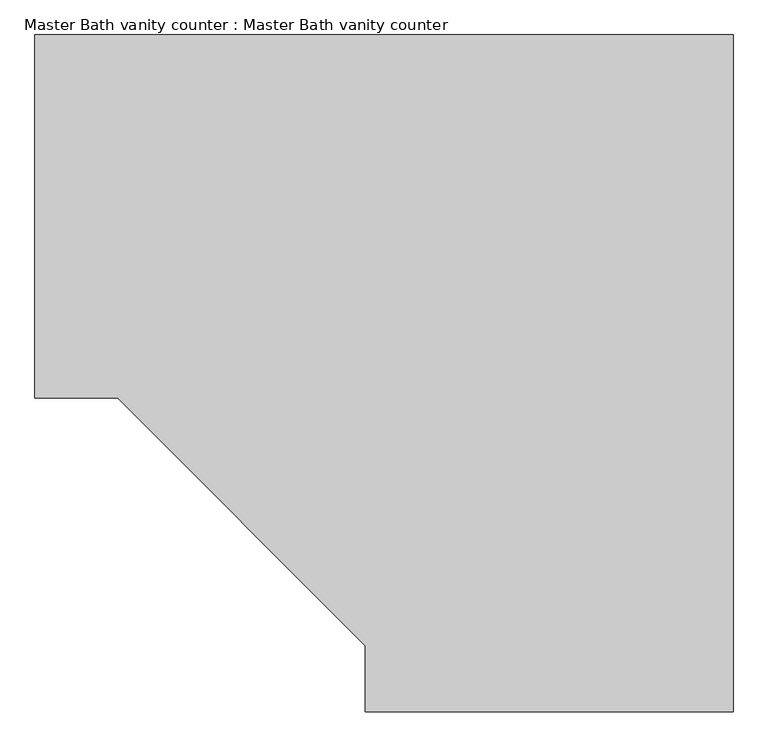
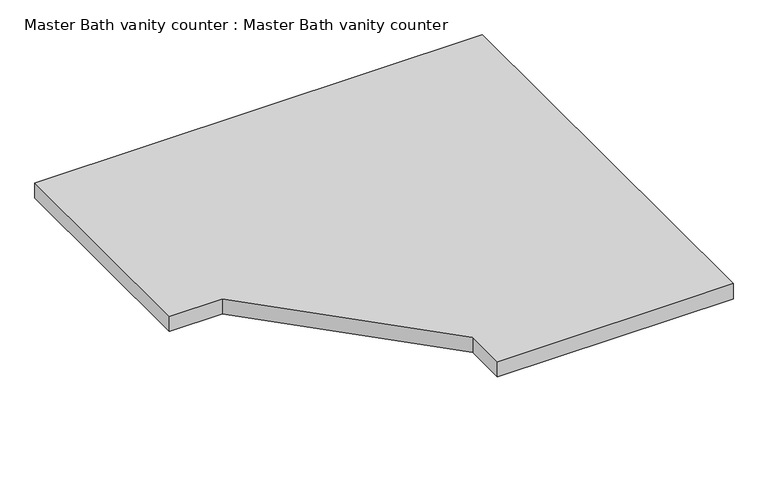
"""IFC4 building model written with IfcOpenShell, lengths in millimetres: furniture geometry, Master Bath vanity counter : Master Bath vanity counter."""

from ifc_helpers import new_model, si_unit, frame, origin, place, context, project, spatial, polyline, outline, extrude, source, transform, mapped, element, save


def master_bath_vanity_counter_master_bath_vanity_counter_6bfa3f7b(model_context):
    return source(origin(), model_context, "Body", "SweptSolid", [
        extrude(outline(polyline([(-7278.6875, 15727.3625), (-6205.5375, 15727.3625), (-6205.5375, 14685.9625), (-6770.6875, 14685.9625), (-6770.6875, 14787.5625), (-7151.6875, 15168.5625), (-7278.6875, 15168.5625), (-7278.6875, 15727.3625)])), frame((0.0, 0.0, 647.7), z_axis=(0.0, 0.0, 1.0), x_axis=(1.0, 0.0, 0.0)), (0.0, 0.0, 1.0), 38.1),
    ])


if __name__ == "__main__":
    model = new_model("IFC4")
    model_context = context("Model", 3, world=origin())
    ifc_project = project(units=[si_unit("LENGTHUNIT", "METRE", prefix="MILLI")], contexts=[model_context])
    site = spatial("IfcSite", under=ifc_project)
    building = spatial("IfcBuilding", under=site)
    placement = place(None, origin())
    master_bath_vanity_counter_master_bath_vanity_counter_shape = master_bath_vanity_counter_master_bath_vanity_counter_6bfa3f7b(model_context)
    element("IfcFurniture", 1, ObjectType="Master Bath vanity counter : Master Bath vanity counter", at=placement, inside=building, context=model_context, shape_type="MappedRepresentation", body=[
        mapped(master_bath_vanity_counter_master_bath_vanity_counter_shape, transform((0.0, 0.0, 0.0), x_axis=(1.0, 0.0, 0.0), y_axis=(0.0, 1.0, 0.0), z_axis=(0.0, 0.0, 1.0))),
    ])
    save(model, "model.ifc")

# Revit data of these elements
# Type "Master Bath vanity counter : Master Bath vanity counter"
#   COBie.Type = no
# Element 1 (IfcFurniture, "Master Bath vanity counter : Master Bath vanity counter")
#   Materials on its faces: "Corian - Emerald"
# Materials
#   "Corian - Emerald": class "Plastic", colour RGB 51 95 44, transparency 0, Cost = 0
